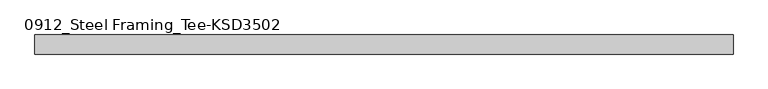
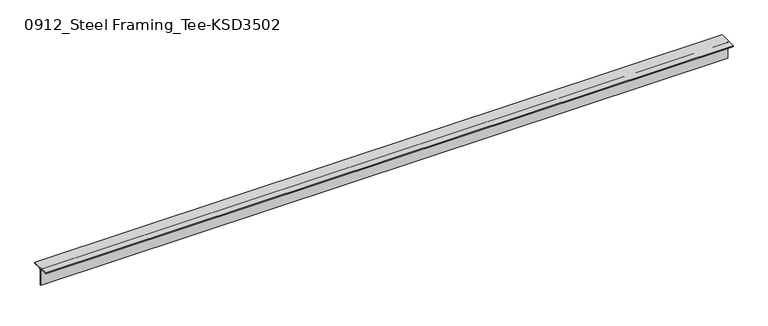
"""IFC4 building model written with IfcOpenShell, lengths in millimetres: member geometry, 0912_Steel Framing_Tee-KSD3502 : H_SB_ASB_CT-150x150x6.5x9."""

import ifcopenshell
import ifcopenshell.guid

model = None  # the IFC model being written
_history = None  # IfcOwnerHistory: only IFC2X3 demands one
_inside = {}  # id of a spatial element -> (the spatial element, [elements in it])
_under = {}  # id of a project, library or spatial element -> (it, [spatial elements below it])
_declared = {}  # id of a project -> (the project, [libraries it declares])
_typed = {}  # id of a type object -> (the type object, [elements of that type])
_made_of = {}  # id of a material, layer set ... -> (it, [elements and type objects made of it])


def new_model(schema):
    """Start an empty IFC model of exactly this schema.

    Asked for "IFC4X3", IfcOpenShell would pick the latest addendum, in which some entities
    have other attributes; the version numbers below select the first issue.
    IFC2X3 requires an IfcOwnerHistory on every rooted entity: one is made here for all.
    """
    global model, _history
    if schema == "IFC4X3":
        model = ifcopenshell.file(schema_version=(4, 3, 0, 0))
    else:
        model = ifcopenshell.file(schema=schema)
    _inside.clear()
    _under.clear()
    _declared.clear()
    _typed.clear()
    _made_of.clear()
    _history = None
    if model.schema == "IFC2X3":
        org = make("IfcOrganization", Name="unknown")
        user = make(
            "IfcPersonAndOrganization",
            ThePerson=make("IfcPerson", FamilyName="unknown"),
            TheOrganization=org,
        )
        app = make(
            "IfcApplication",
            ApplicationDeveloper=org,
            Version="unknown",
            ApplicationFullName="unknown",
            ApplicationIdentifier="unknown",
        )
        _history = make(
            "IfcOwnerHistory",
            OwningUser=user,
            OwningApplication=app,
            ChangeAction="ADDED",
            CreationDate=0,
        )
    return model


def make(cls, **values):
    """One entity of the class cls with the attributes given. An attribute that is None is left unset."""
    return model.create_entity(
        cls, **{name: value for name, value in values.items() if value is not None}
    )


def rooted(cls, **values):
    """An entity with a GlobalId (a new one), such as an element, a storey or a relation."""
    return make(cls, GlobalId=ifcopenshell.guid.new(), OwnerHistory=_history, **values)


def si_unit(unit_type, name, prefix=None):
    """IfcSIUnit, for example si_unit("LENGTHUNIT", "METRE", prefix="MILLI")."""
    return make("IfcSIUnit", UnitType=unit_type, Prefix=prefix, Name=name)


def assignment(units):
    """IfcUnitAssignment: the units of a project."""
    return None if units is None else make("IfcUnitAssignment", Units=units)


def point(xyz):
    """IfcCartesianPoint."""
    return None if xyz is None else make("IfcCartesianPoint", Coordinates=xyz)


def direction(xyz):
    """IfcDirection."""
    return None if xyz is None else make("IfcDirection", DirectionRatios=xyz)


def frame(location, z_axis=None, x_axis=None):
    """IfcAxis2Placement3D, a coordinate frame: its origin and axes. An axis left out is left unset."""
    return make(
        "IfcAxis2Placement3D",
        Location=point(location),
        Axis=direction(z_axis),
        RefDirection=direction(x_axis),
    )


def frame_2d(location, x_axis=None):
    """IfcAxis2Placement2D, a coordinate frame in the plane: its origin and x axis."""
    return make(
        "IfcAxis2Placement2D", Location=point(location), RefDirection=direction(x_axis)
    )


def origin():
    """The frame at (0, 0, 0) with its axes left unset."""
    return frame((0.0, 0.0, 0.0))


def place(relative_to, where):
    """IfcLocalPlacement: puts the frame where relative to a parent placement (None: the world)."""
    return make(
        "IfcLocalPlacement", PlacementRelTo=relative_to, RelativePlacement=where
    )


def context(
    kind, dimensions, precision=None, world=None, true_north=None, identifier=None
):
    """IfcGeometricRepresentationContext, for example the 3D "Model" context."""
    return make(
        "IfcGeometricRepresentationContext",
        ContextIdentifier=identifier,
        ContextType=kind,
        CoordinateSpaceDimension=dimensions,
        Precision=precision,
        WorldCoordinateSystem=world,
        TrueNorth=true_north,
    )


def project(units=None, contexts=None):
    """IfcProject with its units and contexts."""
    return rooted(
        "IfcProject",
        Name="project",
        RepresentationContexts=contexts,
        UnitsInContext=assignment(units),
    )


def spatial(cls, under=None, at=None, **own):
    """A site, building, storey or space (cls), placed at a placement, below another one or the project."""
    s = rooted(cls, ObjectPlacement=at, **own)
    if under is not None:
        _under.setdefault(under.id(), (under, []))[1].append(s)
    return s


def polyline(points):
    """IfcPolyline through the points."""
    return make("IfcPolyline", Points=[point(p) for p in points])


def circle_curve(where, radius):
    """IfcCircle in the frame where."""
    return make("IfcCircle", Position=where, Radius=radius)


def trimmed(basis, trim1, trim2, sense, master):
    """IfcTrimmedCurve: the piece of a basis curve between two trims."""
    return make(
        "IfcTrimmedCurve",
        BasisCurve=basis,
        Trim1=trim1,
        Trim2=trim2,
        SenseAgreement=sense,
        MasterRepresentation=master,
    )


def segment(curve, same_sense, transition):
    """IfcCompositeCurveSegment."""
    return make(
        "IfcCompositeCurveSegment",
        Transition=transition,
        SameSense=same_sense,
        ParentCurve=curve,
    )


def composite_curve(segments, self_intersect=None):
    """IfcCompositeCurve: segments joined end to end."""
    return make("IfcCompositeCurve", Segments=segments, SelfIntersect=self_intersect)


def outline(outer, holes=None, kind="AREA"):
    """IfcArbitraryClosedProfileDef: a profile drawn as a closed curve; with holes, ...WithVoids."""
    if holes is None:
        return make("IfcArbitraryClosedProfileDef", ProfileType=kind, OuterCurve=outer)
    return make(
        "IfcArbitraryProfileDefWithVoids",
        ProfileType=kind,
        OuterCurve=outer,
        InnerCurves=holes,
    )


def extrude(swept, where, along, depth):
    """IfcExtrudedAreaSolid: the profile swept, set in the frame where, extruded along a direction by depth."""
    return make(
        "IfcExtrudedAreaSolid",
        SweptArea=swept,
        Position=where,
        ExtrudedDirection=direction(along),
        Depth=depth,
    )


def shape(context_of_items, identifier, shape_type, items):
    """IfcShapeRepresentation: the items that make up one representation, for example the "Body"."""
    return make(
        "IfcShapeRepresentation",
        ContextOfItems=context_of_items,
        RepresentationIdentifier=identifier,
        RepresentationType=shape_type,
        Items=items,
    )


def source(mapping_origin, context_of_items, identifier, shape_type, items):
    """IfcRepresentationMap: a shape defined once, which mapped items show again and again."""
    return make(
        "IfcRepresentationMap",
        MappingOrigin=mapping_origin,
        MappedRepresentation=shape(context_of_items, identifier, shape_type, items),
    )


def transform(
    local_origin,
    x_axis=None,
    y_axis=None,
    z_axis=None,
    scale=None,
    scale2=None,
    scale3=None,
    uniform=True,
):
    """IfcCartesianTransformationOperator3D, or its non-uniform kind. x_axis, y_axis, z_axis: its Axis1, 2, 3."""
    if uniform:
        return make(
            "IfcCartesianTransformationOperator3D",
            Axis1=direction(x_axis),
            Axis2=direction(y_axis),
            LocalOrigin=point(local_origin),
            Scale=scale,
            Axis3=direction(z_axis),
        )
    return make(
        "IfcCartesianTransformationOperator3DnonUniform",
        Axis1=direction(x_axis),
        Axis2=direction(y_axis),
        LocalOrigin=point(local_origin),
        Scale=scale,
        Axis3=direction(z_axis),
        Scale2=scale2,
        Scale3=scale3,
    )


def mapped(mapping_source, mapping_target):
    """IfcMappedItem: shows the shape of a source again, moved by a transform."""
    return make(
        "IfcMappedItem", MappingSource=mapping_source, MappingTarget=mapping_target
    )


def made_of(thing, what):
    """Note that an element or type object is made of a material, layer set ...; save() writes the relation."""
    if what is not None:
        _made_of.setdefault(what.id(), (what, []))[1].append(thing)
    return thing


def element(
    cls,
    number,
    at=None,
    inside=None,
    cuts=None,
    type_object=None,
    material=None,
    context=None,
    identifier="Body",
    shape_type=None,
    held_by="IfcProductDefinitionShape",
    body=None,
    shapes=None,
    **own,
):
    """One element of the class cls, such as IfcWall. Its Tag is "e" and its number.

    at: its placement. inside: the storey or other place that contains it. cuts: it is an
    opening in that element (IfcRelVoidsElement). A single representation is given by context,
    identifier, shape_type and body (its items); several are given by shapes. held_by: the class
    of the entity that holds the representations. save() writes the other relations.
    """
    e = rooted(cls, Tag="e%d" % number, ObjectPlacement=at, **own)
    if body is not None:
        shapes = [shape(context, identifier, shape_type, body)]
    if shapes is not None:
        e.Representation = make(held_by, Representations=shapes)
    if inside is not None:
        _inside.setdefault(inside.id(), (inside, []))[1].append(e)
    if cuts is not None:
        rooted(
            "IfcRelVoidsElement", RelatingBuildingElement=cuts, RelatedOpeningElement=e
        )
    if type_object is not None:
        _typed.setdefault(type_object.id(), (type_object, []))[1].append(e)
    return made_of(e, material)


def aggregate(whole, parts):
    """IfcRelAggregates: a whole, such as a stair, and the parts it consists of."""
    return rooted("IfcRelAggregates", RelatingObject=whole, RelatedObjects=parts)


def save(model, path):
    """Write the relations noted so far, then the file.

    IfcRelAggregates (storeys below a building ...), IfcRelContainedInSpatialStructure (elements
    in a storey), IfcRelDefinesByType, IfcRelAssociatesMaterial and IfcRelDeclares: one each for
    every whole, place, type object, material and project.
    """
    for whole, parts in _under.values():
        aggregate(whole, parts)
    for where, things in _inside.values():
        rooted(
            "IfcRelContainedInSpatialStructure",
            RelatedElements=things,
            RelatingStructure=where,
        )
    for kind, things in _typed.values():
        rooted("IfcRelDefinesByType", RelatedObjects=things, RelatingType=kind)
    for what, things in _made_of.values():
        rooted("IfcRelAssociatesMaterial", RelatedObjects=things, RelatingMaterial=what)
    for by, libraries in _declared.values():
        rooted("IfcRelDeclares", RelatingContext=by, RelatedDefinitions=libraries)
    model.write(path)


def member_0912_steel_framing_tee_ksd3502_4ae31745(model_context):
    return source(origin(), model_context, "Body", "SweptSolid", [
        extrude(outline(composite_curve([segment(polyline([(-75.0, 75.0), (75.0, 75.0), (75.0, 66.0), (16.25, 66.0)]), True, "CONTINUOUS"), segment(trimmed(circle_curve(frame_2d((16.25, 53.0)), 13.0), [point((16.25, 66.0))], [point((3.25, 53.0))], True, "CARTESIAN"), True, "CONTINUOUS"), segment(polyline([(3.25, 53.0), (3.25, -75.0), (-3.25, -75.0), (-3.25, 53.0)]), True, "CONTINUOUS"), segment(trimmed(circle_curve(frame_2d((-16.25, 53.0)), 13.0), [point((-3.25, 53.0))], [point((-16.25, 66.0))], True, "CARTESIAN"), True, "CONTINUOUS"), segment(polyline([(-16.25, 66.0), (-75.0, 66.0), (-75.0, 75.0)]), True, "CONTINUOUS")], self_intersect=False)), frame((-2735.5, 0.0, 0.0), z_axis=(1.0, 0.0, 0.0), x_axis=(0.0, 1.0, 0.0)), (0.0, 0.0, 1.0), 5478.5),
    ])


if __name__ == "__main__":
    model = new_model("IFC4")
    model_context = context("Model", 3, world=origin())
    ifc_project = project(units=[si_unit("LENGTHUNIT", "METRE", prefix="MILLI")], contexts=[model_context])
    site = spatial("IfcSite", under=ifc_project)
    building = spatial("IfcBuilding", under=site)
    placement = place(None, origin())
    member_0912_steel_framing_tee_ksd3502_shape = member_0912_steel_framing_tee_ksd3502_4ae31745(model_context)
    element("IfcMember", 1, ObjectType="0912_Steel Framing_Tee-KSD3502 : H_SB_ASB_CT-150x150x6.5x9", at=placement, inside=building, context=model_context, shape_type="MappedRepresentation", body=[
        mapped(member_0912_steel_framing_tee_ksd3502_shape, transform((0.0, 0.0, 0.0), x_axis=(1.0, 0.0, 0.0), y_axis=(0.0, 1.0, 0.0), z_axis=(0.0, 0.0, 1.0))),
    ])
    save(model, "model.ifc")

# Revit data of these elements
# Type "0912_Steel Framing_Tee-KSD3502 : H_SB_ASB_CT-150x150x6.5x9"
#   H_WM Code_1 = "S01AA003-00001 | Main Steel Structure Fabrication Work | Shelter/Building | Light Steel - Standard (30KG/M>Weight) | Material: (   )"
#   H_WM Code_2 = "S03AA029-00001 | Main Steel Structure Erection Work | Shelter/Building | Light Steel (30KG/M>Weight) | Material: (   )"
#   H_WM Code_3 = "S01AA010-00001 | Main Steel Structure Fabrication Work | Shelter/Building | Steel Painting/Coating | for Non-Fireproofed Steel Surface, Surface Preparation, Primer, Second & Final Coat | Material: (   )"
#   H_Q'ty Cal Type Tag = "SB-Q2"
#   Width = 15.0 cm
#   Web Thickness = 0.65 cm
#   Web Fillet = 1.3 cm
#   Section Area = 23.39 cm²
#   Perimeter = 0.60 m²/m
#   Nominal Weight = 18.40 kgf/m
#   Height = 15.0 cm
#   Flange Thickness = 0.9 cm
#   Centroid Vertical = 7.5 cm
#   Centroid Horizontal = 7.5 cm
#   Length [instance default] = 1.5000 m
#   Structural Material [instance default] = Steel, 45-345
#   Warping Constant = (empty or 0)
#   Torsional Moment of Inertia = 0
#   Section Name Key = ""
#   Plastic Modulus weak axis = 0
#   Plastic Modulus strong axis = 0
#   Moment of Inertia weak axis = 0
#   Moment of Inertia strong axis = 0
#   Elastic Modulus weak axis = 0
#   Elastic Modulus strong axis = 0
#   Bolt Spacing = 0
#   Assembly Code = ""
# Element 1 (IfcMember, "0912_Steel Framing_Tee-KSD3502 : H_SB_ASB_CT-150x150x6.5x9")
#   Structural Material = none
# Materials
#   "Steel, 45-345": class "Metal", colour RGB 189 187 185, transparency 0, Description = "Steel 345 MPa", Cost = 0
